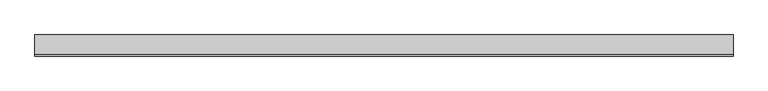
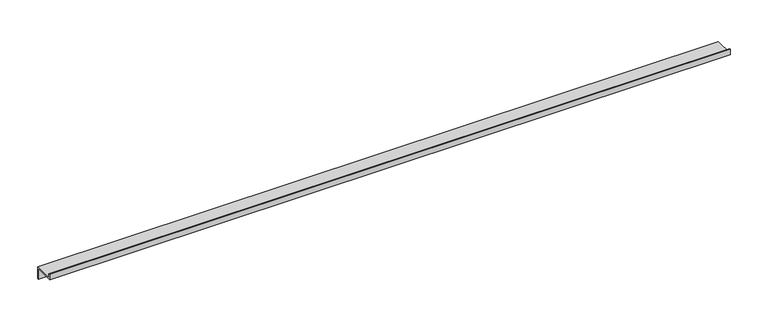
"""IFC4 building model written with IfcOpenShell, lengths in millimetres: proxy geometry, Generic Models 7:Generic Models 1:7:Generic Models 1:7 : Generic Models 7:Generic Models 1:337419:1 : Generic Models 7:Generic Models 1:7:Generic Models 1:7 : Generic Models 7:Generic Models 1:337419:315055."""

from ifc_helpers import new_model, si_unit, frame, origin, place, context, project, spatial, polyline, outline, extrude, source, transform, mapped, element, save


def generic_models_c6bc166c(model_context):
    return source(origin(), model_context, "Body", "SweptSolid", [
        extrude(outline(polyline([(-579020.0498787, 9.6477948), (-579020.0498787, 26.9875), (-579050.0551409, 26.9875), (-579050.0551409, 35.3140132), (-579048.4676409, 35.3140132), (-579048.4676409, 28.575), (-579018.4623787, 28.575), (-579018.4623787, 9.6477948), (-579020.0498787, 9.6477948)])), frame((591714.0570845, 0.0, 0.0), z_axis=(1.0, 0.0, 0.0), x_axis=(0.0, 1.0, 0.0)), (0.0, 0.0, 1.0), 1044.8567691),
    ])


if __name__ == "__main__":
    model = new_model("IFC4")
    model_context = context("Model", 3, world=origin())
    ifc_project = project(units=[si_unit("LENGTHUNIT", "METRE", prefix="MILLI")], contexts=[model_context])
    site = spatial("IfcSite", under=ifc_project)
    building = spatial("IfcBuilding", under=site)
    placement = place(None, origin())
    generic_models_shape = generic_models_c6bc166c(model_context)
    element("IfcBuildingElementProxy", 1, Name="Generic Models 7:Generic Models 1:7:Generic Models 1:7 : Generic Models 7:Generic Models 1:337419:1 : Generic Models 7:Generic Models 1:7:Generic Models 1:7 : Generic Models 7:Generic Models 1:337419:315055", ObjectType="Generic Models 7:Generic Models 1:7:Generic Models 1:7 : Generic Models 7:Generic Models 1:337419:1 : Generic Models 7:Generic Models 1:7:Generic Models 1:7 : Generic Models 7:Generic Models 1:337419:315055", at=placement, inside=building, context=model_context, shape_type="MappedRepresentation", body=[
        mapped(generic_models_shape, transform((0.0, 0.0, 0.0), x_axis=(1.0, 0.0, 0.0), y_axis=(0.0, 1.0, 0.0), z_axis=(0.0, 0.0, 1.0))),
    ])
    save(model, "model.ifc")

# Revit data of these elements
# Type "Generic Models 7:Generic Models 1:7:Generic Models 1:7 : Generic Models 7:Generic Models 1:337419:1 : Generic Models 7:Generic Models 1:7:Generic Models 1:7 : Generic Models 7:Generic Models 1:337419:315055"
#   NameOverride = "Generic Models 7:Generic Models 1:7:Generic Models 1:7 : Generic Models 7:Generic Models 1:337419:315055"
#   ObjectTypeOverride = "Generic Models 1:7 : Generic Models 7:Generic Models 1:337419"
#   Reference = "Generic Models 1"
#   Tag = "315055"
# Element 1 (IfcBuildingElementProxy, "Generic Models 7:Generic Models 1:7:Generic Models 1:7 : Generic Models 7:Generic Models 1:337419:1 : Generic Models 7:Generic Models 1:7:Generic Models 1:7 : Generic Models 7:Generic Models 1:337419:315055")
#   Materials on its faces: "STAINLESS STEEL BENT PLATE (FLASHING)"
# Materials
#   "STAINLESS STEEL BENT PLATE (FLASHING)": class "Unassigned", colour RGB 210 209 208, transparency 0, Cost = 0
